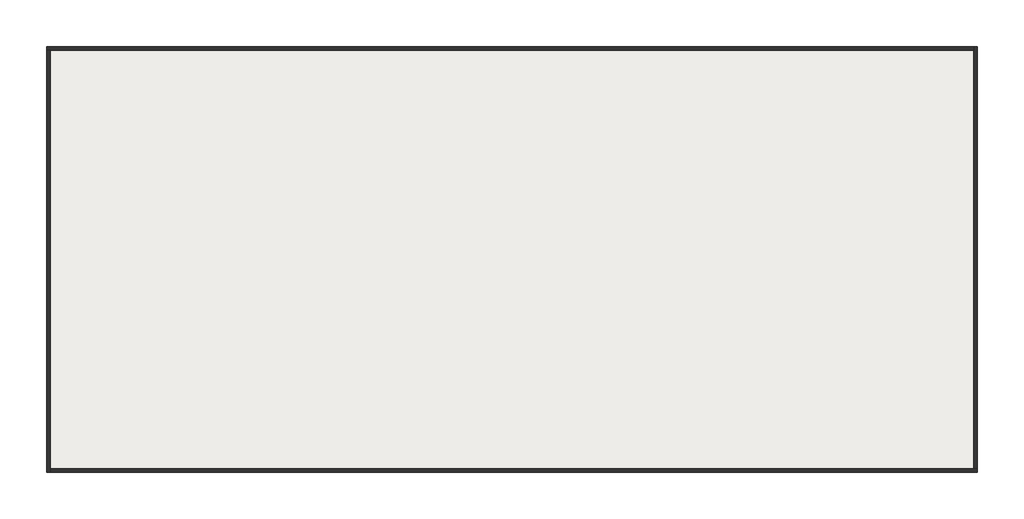
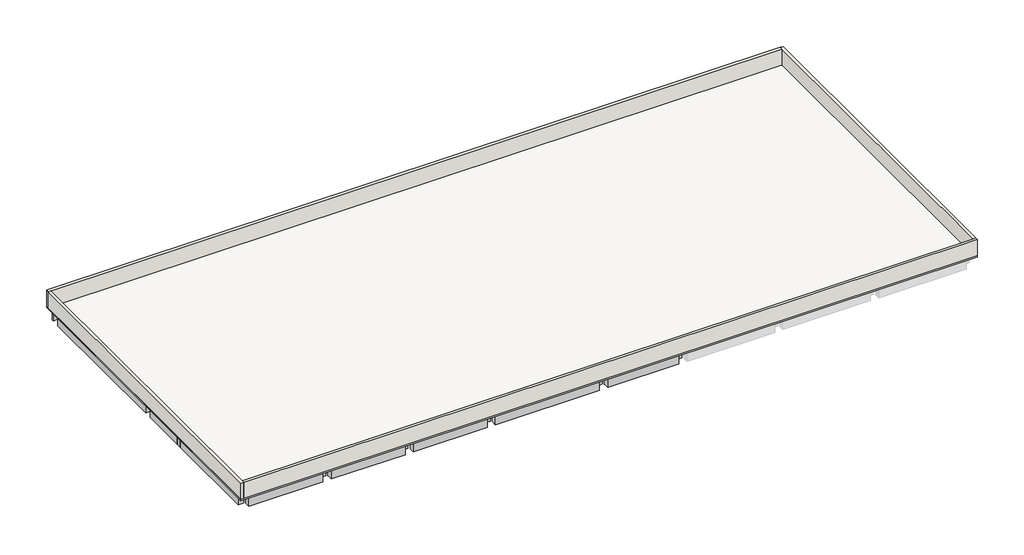
# One storey, part 1 of 2: 33 beams, 4 walls, 1 roof.
"""IFC4 building model written with IfcOpenShell, lengths in millimetres."""

from ifc_helpers import new_model, si_unit, frame, origin, place, context, project, spatial, polyline, outline, extrude, faceted_brep, element, save

model = new_model("IFC4")

# Units and contexts
model_context = context("Model", 3, world=origin())
ifc_project = project(units=[si_unit("LENGTHUNIT", "METRE", prefix="MILLI")], contexts=[model_context])

# Site, building, storey
site = spatial("IfcSite", under=ifc_project)
building = spatial("IfcBuilding", under=site)
storey = spatial("IfcBuildingStorey", under=building, Name="TOC", Elevation=7650.0)

# Beams
placement = place(None, origin())
element("IfcBeam", 1, ObjectType="RC Beam_Rectangular : H_SB_ACB_B400xH900", at=placement, inside=storey, context=model_context, shape_type="Brep", body=[
    faceted_brep([(224.7, 12116.5208589, 7500.0), (224.7, 12116.5208589, 6750.0), (5624.7, 12116.5208589, 6750.0), (5624.7, 12116.5208589, 7500.0), (5724.7, 12116.5208589, 7500.0), (6124.7, 12116.5208589, 7500.0), (6124.7, 12116.5208589, 7549.0), (5724.7, 12116.5208589, 7549.0), (124.7, 12116.5208589, 7549.0), (-275.3, 12116.5208589, 7549.0), (-275.3, 12116.5208589, 7500.0), (124.7, 12116.5208589, 7500.0), (224.7, 12199.5208589, 6750.0), (224.7, 12433.5208589, 6750.0), (224.7, 12516.5208589, 6750.0), (5624.7, 12516.5208589, 6750.0), (5624.7, 12433.5208589, 6750.0), (5624.7, 12199.5208589, 6750.0), (224.7, 12516.5208589, 7500.0), (124.7, 12516.5208589, 7500.0), (-275.3, 12516.5208589, 7500.0), (-275.3, 12516.5208589, 7549.0), (124.7, 12516.5208589, 7549.0), (5724.7, 12516.5208589, 7549.0), (6124.7, 12516.5208589, 7549.0), (6124.7, 12516.5208589, 7500.0), (5724.7, 12516.5208589, 7500.0), (5624.7, 12516.5208589, 7500.0)], [[[0, 1, 2, 3, 4, 5, 6, 7, 8, 9, 10, 11]], [[1, 12, 13, 14, 15, 16, 17, 2]], [[14, 18, 19, 20, 21, 22, 23, 24, 25, 26, 27, 15]], [[1, 0, 18, 14, 13, 12]], [[0, 11, 10, 20, 19, 18]], [[27, 3, 2, 17, 16, 15]], [[3, 27, 26, 25, 5, 4]], [[9, 8, 7, 6, 24, 23, 22, 21]], [[9, 21, 20, 10]], [[24, 6, 5, 25]]]),
])
element("IfcBeam", 2, ObjectType="RC Beam_Rectangular : H_SB_ACB_B400xH900", at=placement, inside=storey, context=model_context, shape_type="Brep", body=[
    faceted_brep([(6224.7, 12116.5208589, 7500.0), (6224.7, 12116.5208589, 6750.0), (11624.7, 12116.5208589, 6750.0), (11624.7, 12116.5208589, 7500.0), (11724.7, 12116.5208589, 7500.0), (12124.7, 12116.5208589, 7500.0), (12124.7, 12116.5208589, 7549.0), (11724.7, 12116.5208589, 7549.0), (6124.7, 12116.5208589, 7549.0), (6124.7, 12116.5208589, 7500.0), (6224.7, 12199.5208589, 6750.0), (6224.7, 12433.5208589, 6750.0), (6224.7, 12516.5208589, 6750.0), (11624.7, 12516.5208589, 6750.0), (11624.7, 12433.5208589, 6750.0), (11624.7, 12199.5208589, 6750.0), (6224.7, 12516.5208589, 7500.0), (6124.7, 12516.5208589, 7500.0), (6124.7, 12516.5208589, 7549.0), (11724.7, 12516.5208589, 7549.0), (12124.7, 12516.5208589, 7549.0), (12124.7, 12516.5208589, 7500.0), (11724.7, 12516.5208589, 7500.0), (11624.7, 12516.5208589, 7500.0)], [[[0, 1, 2, 3, 4, 5, 6, 7, 8, 9]], [[1, 10, 11, 12, 13, 14, 15, 2]], [[12, 16, 17, 18, 19, 20, 21, 22, 23, 13]], [[1, 0, 16, 12, 11, 10]], [[0, 9, 17, 16]], [[23, 3, 2, 15, 14, 13]], [[3, 23, 22, 21, 5, 4]], [[8, 7, 6, 20, 19, 18]], [[20, 6, 5, 21]], [[8, 18, 17, 9]]]),
])
element("IfcBeam", 3, ObjectType="RC Beam_Rectangular : H_SB_ACB_B400xH900", at=placement, inside=storey, context=model_context, shape_type="Brep", body=[
    faceted_brep([(12224.7, 12116.5208589, 7500.0), (12224.7, 12116.5208589, 6750.0), (17624.7, 12116.5208589, 6750.0), (17624.7, 12116.5208589, 7500.0), (17724.7, 12116.5208589, 7500.0), (18124.7, 12116.5208589, 7500.0), (18124.7, 12116.5208589, 7549.0), (17724.7, 12116.5208589, 7549.0), (12124.7, 12116.5208589, 7549.0), (12124.7, 12116.5208589, 7500.0), (12224.7, 12199.5208589, 6750.0), (12224.7, 12433.5208589, 6750.0), (12224.7, 12516.5208589, 6750.0), (17624.7, 12516.5208589, 6750.0), (17624.7, 12433.5208589, 6750.0), (17624.7, 12199.5208589, 6750.0), (12224.7, 12516.5208589, 7500.0), (12124.7, 12516.5208589, 7500.0), (12124.7, 12516.5208589, 7549.0), (17724.7, 12516.5208589, 7549.0), (18124.7, 12516.5208589, 7549.0), (18124.7, 12516.5208589, 7500.0), (17724.7, 12516.5208589, 7500.0), (17624.7, 12516.5208589, 7500.0)], [[[0, 1, 2, 3, 4, 5, 6, 7, 8, 9]], [[1, 10, 11, 12, 13, 14, 15, 2]], [[12, 16, 17, 18, 19, 20, 21, 22, 23, 13]], [[1, 0, 16, 12, 11, 10]], [[0, 9, 17, 16]], [[23, 3, 2, 15, 14, 13]], [[3, 23, 22, 21, 5, 4]], [[8, 7, 6, 20, 19, 18]], [[20, 6, 5, 21]], [[8, 18, 17, 9]]]),
])
element("IfcBeam", 4, ObjectType="RC Beam_Rectangular : H_SB_ACB_B400xH900", at=placement, inside=storey, context=model_context, shape_type="Brep", body=[
    faceted_brep([(26324.7, 12116.5208589, 7549.0), (25924.7, 12116.5208589, 7549.0), (18124.7, 12116.5208589, 7549.0), (18124.7, 12116.5208589, 7500.0), (18224.7, 12116.5208589, 7500.0), (18224.7, 12116.5208589, 6750.0), (25924.7, 12116.5208589, 6750.0), (26324.7, 12116.5208589, 6750.0), (26324.7, 12516.5208589, 6750.0), (18224.7, 12516.5208589, 6750.0), (25924.7, 12516.5208589, 6750.0), (18124.7, 12516.5208589, 7549.0), (25924.7, 12516.5208589, 7549.0), (26324.7, 12516.5208589, 7549.0), (18224.7, 12516.5208589, 7500.0), (18124.7, 12516.5208589, 7500.0)], [[[0, 1, 2, 3, 4, 5, 6, 7]], [[8, 7, 6, 5, 9, 10]], [[11, 12, 13, 8, 10, 9, 14, 15]], [[4, 14, 9, 5]], [[14, 4, 3, 15]], [[2, 1, 0, 13, 12, 11]], [[7, 8, 13, 0]], [[2, 11, 15, 3]]]),
])
element("IfcBeam", 5, ObjectType="RC Beam_Rectangular : H_SB_ACB_B400xH900", at=placement, inside=storey, context=model_context, shape_type="Brep", body=[
    faceted_brep([(32124.7, 12116.5208589, 6750.0), (32124.7, 12116.5208589, 7549.0), (31724.7, 12116.5208589, 7549.0), (26324.7, 12116.5208589, 7549.0), (26324.7, 12116.5208589, 6750.0), (31724.7, 12116.5208589, 6750.0), (32124.7, 12516.5208589, 6750.0), (26324.7, 12516.5208589, 6750.0), (31724.7, 12516.5208589, 6750.0), (32124.7, 12516.5208589, 7549.0), (26324.7, 12516.5208589, 7549.0), (31724.7, 12516.5208589, 7549.0)], [[[0, 1, 2, 3, 4, 5]], [[6, 0, 5, 4, 7, 8]], [[9, 6, 8, 7, 10, 11]], [[1, 9, 11, 10, 3, 2]], [[0, 6, 9, 1]], [[4, 3, 10, 7]]]),
])
element("IfcBeam", 6, ObjectType="RC Beam_Rectangular : H_SB_ACB_B400xH900", at=placement, inside=storey, context=model_context, shape_type="Brep", body=[
    faceted_brep([(224.7, 23816.5208589, 7500.0), (224.7, 23816.5208589, 6750.0), (5624.7, 23816.5208589, 6750.0), (5624.7, 23816.5208589, 7500.0), (5724.7, 23816.5208589, 7500.0), (5724.7, 23816.5208589, 7549.0), (124.7, 23816.5208589, 7549.0), (124.7, 23816.5208589, 7500.0), (224.7, 23886.5208589, 6750.0), (224.7, 24216.5208589, 6750.0), (5624.7, 24216.5208589, 6750.0), (5624.7, 23886.5208589, 6750.0), (224.7, 24216.5208589, 7500.0), (124.7, 24216.5208589, 7500.0), (124.7, 24216.5208589, 7549.0), (5724.7, 24216.5208589, 7549.0), (5724.7, 24216.5208589, 7500.0), (5624.7, 24216.5208589, 7500.0)], [[[0, 1, 2, 3, 4, 5, 6, 7]], [[1, 8, 9, 10, 11, 2]], [[9, 12, 13, 14, 15, 16, 17, 10]], [[1, 0, 12, 9, 8]], [[12, 0, 7, 13]], [[3, 2, 11, 10, 17]], [[3, 17, 16, 4]], [[14, 6, 5, 15]], [[7, 6, 14, 13]], [[5, 4, 16, 15]]]),
])
element("IfcBeam", 7, ObjectType="RC Beam_Rectangular : H_SB_ACB_B400xH900", at=placement, inside=storey, context=model_context, shape_type="Brep", body=[
    faceted_brep([(6224.7, 23816.5208589, 7500.0), (6224.7, 23816.5208589, 6750.0), (11624.7, 23816.5208589, 6750.0), (11624.7, 23816.5208589, 7500.0), (11724.7, 23816.5208589, 7500.0), (11724.7, 23816.5208589, 7549.0), (6124.7, 23816.5208589, 7549.0), (6124.7, 23816.5208589, 7500.0), (6224.7, 23886.5208589, 6750.0), (6224.7, 24216.5208589, 6750.0), (11624.7, 24216.5208589, 6750.0), (11624.7, 23886.5208589, 6750.0), (6224.7, 24216.5208589, 7500.0), (6124.7, 24216.5208589, 7500.0), (6124.7, 24216.5208589, 7549.0), (11724.7, 24216.5208589, 7549.0), (11724.7, 24216.5208589, 7500.0), (11624.7, 24216.5208589, 7500.0)], [[[0, 1, 2, 3, 4, 5, 6, 7]], [[1, 8, 9, 10, 11, 2]], [[9, 12, 13, 14, 15, 16, 17, 10]], [[1, 0, 12, 9, 8]], [[0, 7, 13, 12]], [[3, 2, 11, 10, 17]], [[3, 17, 16, 4]], [[14, 6, 5, 15]], [[6, 14, 13, 7]], [[5, 4, 16, 15]]]),
])
element("IfcBeam", 8, ObjectType="RC Beam_Rectangular : H_SB_ACB_B400xH900", at=placement, inside=storey, context=model_context, shape_type="Brep", body=[
    faceted_brep([(12224.7, 23816.5208589, 7500.0), (12224.7, 23816.5208589, 6750.0), (17624.7, 23816.5208589, 6750.0), (17624.7, 23816.5208589, 7500.0), (17724.7, 23816.5208589, 7500.0), (17724.7, 23816.5208589, 7549.0), (12124.7, 23816.5208589, 7549.0), (12124.7, 23816.5208589, 7500.0), (12224.7, 23886.5208589, 6750.0), (12224.7, 24216.5208589, 6750.0), (17624.7, 24216.5208589, 6750.0), (17624.7, 23886.5208589, 6750.0), (12224.7, 24216.5208589, 7500.0), (12124.7, 24216.5208589, 7500.0), (12124.7, 24216.5208589, 7549.0), (17724.7, 24216.5208589, 7549.0), (17724.7, 24216.5208589, 7500.0), (17624.7, 24216.5208589, 7500.0)], [[[0, 1, 2, 3, 4, 5, 6, 7]], [[1, 8, 9, 10, 11, 2]], [[9, 12, 13, 14, 15, 16, 17, 10]], [[1, 0, 12, 9, 8]], [[0, 7, 13, 12]], [[3, 2, 11, 10, 17]], [[3, 17, 16, 4]], [[14, 6, 5, 15]], [[6, 14, 13, 7]], [[5, 4, 16, 15]]]),
])
element("IfcBeam", 9, ObjectType="RC Beam_Rectangular : H_SB_ACB_B400xH900", at=placement, inside=storey, context=model_context, shape_type="Brep", body=[
    faceted_brep([(-275.3, 8216.5208589, 6750.0), (124.7, 8216.5208589, 6750.0), (5724.7, 8216.5208589, 6750.0), (6124.7, 8216.5208589, 6750.0), (6124.7, 8216.5208589, 7549.0), (5724.7, 8216.5208589, 7549.0), (124.7, 8216.5208589, 7549.0), (-275.3, 8216.5208589, 7549.0), (-275.3, 8616.5208589, 6750.0), (124.7, 8616.5208589, 6750.0), (5724.7, 8616.5208589, 6750.0), (6124.7, 8616.5208589, 6750.0), (-275.3, 8616.5208589, 7549.0), (124.7, 8616.5208589, 7549.0), (5724.7, 8616.5208589, 7549.0), (6124.7, 8616.5208589, 7549.0)], [[[0, 1, 2, 3, 4, 5, 6, 7]], [[0, 8, 9, 10, 11, 3, 2, 1]], [[11, 10, 9, 8, 12, 13, 14, 15]], [[7, 6, 5, 4, 15, 14, 13, 12]], [[8, 0, 7, 12]], [[3, 11, 15, 4]]]),
])
element("IfcBeam", 10, ObjectType="RC Beam_Rectangular : H_SB_ACB_B400xH900", at=placement, inside=storey, context=model_context, shape_type="Brep", body=[
    faceted_brep([(12124.7, 8216.5208589, 6750.0), (12124.7, 8216.5208589, 7549.0), (11724.7, 8216.5208589, 7549.0), (6124.7, 8216.5208589, 7549.0), (6124.7, 8216.5208589, 6750.0), (11724.7, 8216.5208589, 6750.0), (12124.7, 8616.5208589, 6750.0), (6124.7, 8616.5208589, 6750.0), (11724.7, 8616.5208589, 6750.0), (12124.7, 8616.5208589, 7549.0), (6124.7, 8616.5208589, 7549.0), (11724.7, 8616.5208589, 7549.0)], [[[0, 1, 2, 3, 4, 5]], [[6, 0, 5, 4, 7, 8]], [[9, 6, 8, 7, 10, 11]], [[1, 9, 11, 10, 3, 2]], [[0, 6, 9, 1]], [[4, 3, 10, 7]]]),
])
element("IfcBeam", 11, ObjectType="RC Beam_Rectangular : H_SB_ACB_B400xH900", at=placement, inside=storey, context=model_context, shape_type="Brep", body=[
    faceted_brep([(18124.7, 8216.5208589, 6750.0), (18124.7, 8216.5208589, 7549.0), (17724.7, 8216.5208589, 7549.0), (12124.7, 8216.5208589, 7549.0), (12124.7, 8216.5208589, 6750.0), (17724.7, 8216.5208589, 6750.0), (18124.7, 8616.5208589, 6750.0), (12124.7, 8616.5208589, 6750.0), (17724.7, 8616.5208589, 6750.0), (18124.7, 8616.5208589, 7549.0), (12124.7, 8616.5208589, 7549.0), (17724.7, 8616.5208589, 7549.0)], [[[0, 1, 2, 3, 4, 5]], [[6, 0, 5, 4, 7, 8]], [[9, 6, 8, 7, 10, 11]], [[1, 9, 11, 10, 3, 2]], [[0, 6, 9, 1]], [[4, 3, 10, 7]]]),
])
element("IfcBeam", 12, ObjectType="RC Beam_Rectangular : H_SB_ACB_B400xH900", at=placement, inside=storey, context=model_context, shape_type="Brep", body=[
    faceted_brep([(26324.7, 8216.5208589, 7549.0), (25924.7, 8216.5208589, 7549.0), (18124.7, 8216.5208589, 7549.0), (18124.7, 8216.5208589, 6750.0), (25824.7, 8216.5208589, 6750.0), (25824.7, 8216.5208589, 7500.0), (25924.7, 8216.5208589, 7500.0), (26324.7, 8216.5208589, 7500.0), (18124.7, 8616.5208589, 6750.0), (25824.7, 8616.5208589, 6750.0), (25824.7, 8533.5208589, 6750.0), (25824.7, 8299.5208589, 6750.0), (18124.7, 8616.5208589, 7549.0), (25924.7, 8616.5208589, 7549.0), (26324.7, 8616.5208589, 7549.0), (26324.7, 8616.5208589, 7500.0), (25924.7, 8616.5208589, 7500.0), (25824.7, 8616.5208589, 7500.0)], [[[0, 1, 2, 3, 4, 5, 6, 7]], [[3, 8, 9, 10, 11, 4]], [[12, 13, 14, 15, 16, 17, 9, 8]], [[17, 5, 4, 11, 10, 9]], [[5, 17, 16, 15, 7, 6]], [[2, 1, 0, 14, 13, 12]], [[14, 0, 7, 15]], [[3, 2, 12, 8]]]),
])
element("IfcBeam", 13, ObjectType="RC Beam_Rectangular : H_SB_ACB_B400xH900", at=placement, inside=storey, context=model_context, shape_type="Brep", body=[
    faceted_brep([(26424.7, 8216.5208589, 7500.0), (26424.7, 8216.5208589, 6750.0), (28824.7, 8216.5208589, 6750.0), (29058.7, 8216.5208589, 6750.0), (31624.7, 8216.5208589, 6750.0), (31624.7, 8216.5208589, 7500.0), (31724.7, 8216.5208589, 7500.0), (32124.7, 8216.5208589, 7500.0), (32124.7, 8216.5208589, 7549.0), (31724.7, 8216.5208589, 7549.0), (31624.7, 8216.5208589, 7549.0), (29058.7, 8216.5208589, 7549.0), (28824.7, 8216.5208589, 7549.0), (26424.7, 8216.5208589, 7549.0), (26324.7, 8216.5208589, 7549.0), (26324.7, 8216.5208589, 7500.0), (26424.7, 8299.5208589, 6750.0), (26424.7, 8533.5208589, 6750.0), (26424.7, 8616.5208589, 6750.0), (31624.7, 8616.5208589, 6750.0), (31624.7, 8533.5208589, 6750.0), (31624.7, 8299.5208589, 6750.0), (26424.7, 8616.5208589, 7500.0), (26324.7, 8616.5208589, 7500.0), (26324.7, 8616.5208589, 7549.0), (31724.7, 8616.5208589, 7549.0), (32124.7, 8616.5208589, 7549.0), (32124.7, 8616.5208589, 7500.0), (31724.7, 8616.5208589, 7500.0), (31624.7, 8616.5208589, 7500.0)], [[[0, 1, 2, 3, 4, 5, 6, 7, 8, 9, 10, 11, 12, 13, 14, 15]], [[1, 16, 17, 18, 19, 20, 21, 4, 3, 2]], [[18, 22, 23, 24, 25, 26, 27, 28, 29, 19]], [[1, 0, 22, 18, 17, 16]], [[0, 15, 23, 22]], [[29, 5, 4, 21, 20, 19]], [[5, 29, 28, 27, 7, 6]], [[14, 13, 12, 11, 10, 9, 8, 26, 25, 24]], [[26, 8, 7, 27]], [[14, 24, 23, 15]]]),
])
element("IfcBeam", 14, ObjectType="RC Beam_Rectangular : H_SB_ACB_B400xH900", at=placement, inside=storey, context=model_context, shape_type="Brep", body=[
    faceted_brep([(224.7, 416.5208589, 7500.0), (224.7, 416.5208589, 6750.0), (5624.7, 416.5208589, 6750.0), (5624.7, 416.5208589, 7500.0), (6124.7, 416.5208589, 7500.0), (6124.7, 416.5208589, 7549.0), (54.7, 416.5208589, 7549.0), (-275.3, 416.5208589, 7549.0), (-275.3, 416.5208589, 7500.0), (54.7, 416.5208589, 7500.0), (224.7, 746.5208589, 6750.0), (224.7, 816.5208589, 6750.0), (5624.7, 816.5208589, 6750.0), (5624.7, 746.5208589, 6750.0), (224.7, 816.5208589, 7500.0), (124.7, 816.5208589, 7500.0), (-275.3, 816.5208589, 7500.0), (-275.3, 816.5208589, 7549.0), (124.7, 816.5208589, 7549.0), (5724.7, 816.5208589, 7549.0), (6124.7, 816.5208589, 7549.0), (6124.7, 816.5208589, 7500.0), (5724.7, 816.5208589, 7500.0), (5624.7, 816.5208589, 7500.0)], [[[0, 1, 2, 3, 4, 5, 6, 7, 8, 9]], [[1, 10, 11, 12, 13, 2]], [[11, 14, 15, 16, 17, 18, 19, 20, 21, 22, 23, 12]], [[11, 10, 1, 0, 14]], [[16, 15, 14, 0, 9, 8]], [[23, 3, 2, 13, 12]], [[3, 23, 22, 21, 4]], [[7, 6, 5, 20, 19, 18, 17]], [[7, 17, 16, 8]], [[20, 5, 4, 21]]]),
])
element("IfcBeam", 15, ObjectType="RC Beam_Rectangular : H_SB_ACB_B400xH900", at=placement, inside=storey, context=model_context, shape_type="Brep", body=[
    faceted_brep([(6224.7, 416.5208589, 7500.0), (6224.7, 416.5208589, 6750.0), (11624.7, 416.5208589, 6750.0), (11624.7, 416.5208589, 7500.0), (12124.7, 416.5208589, 7500.0), (12124.7, 416.5208589, 7549.0), (6124.7, 416.5208589, 7549.0), (6124.7, 416.5208589, 7500.0), (6224.7, 746.5208589, 6750.0), (6224.7, 816.5208589, 6750.0), (11624.7, 816.5208589, 6750.0), (11624.7, 746.5208589, 6750.0), (6224.7, 816.5208589, 7500.0), (6124.7, 816.5208589, 7500.0), (6124.7, 816.5208589, 7549.0), (11724.7, 816.5208589, 7549.0), (12124.7, 816.5208589, 7549.0), (12124.7, 816.5208589, 7500.0), (11724.7, 816.5208589, 7500.0), (11624.7, 816.5208589, 7500.0)], [[[0, 1, 2, 3, 4, 5, 6, 7]], [[1, 8, 9, 10, 11, 2]], [[9, 12, 13, 14, 15, 16, 17, 18, 19, 10]], [[9, 8, 1, 0, 12]], [[13, 12, 0, 7]], [[19, 3, 2, 11, 10]], [[3, 19, 18, 17, 4]], [[6, 5, 16, 15, 14]], [[16, 5, 4, 17]], [[6, 14, 13, 7]]]),
])
element("IfcBeam", 16, ObjectType="RC Beam_Rectangular : H_SB_ACB_B400xH900", at=placement, inside=storey, context=model_context, shape_type="Brep", body=[
    faceted_brep([(12224.7, 416.5208589, 7500.0), (12224.7, 416.5208589, 6750.0), (17624.7, 416.5208589, 6750.0), (17624.7, 416.5208589, 7500.0), (18124.7, 416.5208589, 7500.0), (18124.7, 416.5208589, 7549.0), (12124.7, 416.5208589, 7549.0), (12124.7, 416.5208589, 7500.0), (12224.7, 746.5208589, 6750.0), (12224.7, 816.5208589, 6750.0), (17624.7, 816.5208589, 6750.0), (17624.7, 746.5208589, 6750.0), (12224.7, 816.5208589, 7500.0), (12124.7, 816.5208589, 7500.0), (12124.7, 816.5208589, 7549.0), (17724.7, 816.5208589, 7549.0), (18124.7, 816.5208589, 7549.0), (18124.7, 816.5208589, 7500.0), (17724.7, 816.5208589, 7500.0), (17624.7, 816.5208589, 7500.0)], [[[0, 1, 2, 3, 4, 5, 6, 7]], [[1, 8, 9, 10, 11, 2]], [[9, 12, 13, 14, 15, 16, 17, 18, 19, 10]], [[9, 8, 1, 0, 12]], [[13, 12, 0, 7]], [[19, 3, 2, 11, 10]], [[3, 19, 18, 17, 4]], [[6, 5, 16, 15, 14]], [[16, 5, 4, 17]], [[6, 14, 13, 7]]]),
])
element("IfcBeam", 17, ObjectType="RC Beam_Rectangular : H_SB_ACB_B400xH900", at=placement, inside=storey, context=model_context, shape_type="Brep", body=[
    faceted_brep([(18224.7, 416.5208589, 7500.0), (18224.7, 416.5208589, 6750.0), (25824.7, 416.5208589, 6750.0), (25824.7, 416.5208589, 7500.0), (26324.7, 416.5208589, 7500.0), (26324.7, 416.5208589, 7549.0), (18124.7, 416.5208589, 7549.0), (18124.7, 416.5208589, 7500.0), (18224.7, 746.5208589, 6750.0), (18224.7, 816.5208589, 6750.0), (25824.7, 816.5208589, 6750.0), (25824.7, 746.5208589, 6750.0), (18224.7, 816.5208589, 7500.0), (18124.7, 816.5208589, 7500.0), (18124.7, 816.5208589, 7549.0), (25924.7, 816.5208589, 7549.0), (26324.7, 816.5208589, 7549.0), (26324.7, 816.5208589, 7500.0), (25924.7, 816.5208589, 7500.0), (25824.7, 816.5208589, 7500.0)], [[[0, 1, 2, 3, 4, 5, 6, 7]], [[1, 8, 9, 10, 11, 2]], [[9, 12, 13, 14, 15, 16, 17, 18, 19, 10]], [[9, 8, 1, 0, 12]], [[13, 12, 0, 7]], [[19, 3, 2, 11, 10]], [[3, 19, 18, 17, 4]], [[6, 5, 16, 15, 14]], [[16, 5, 4, 17]], [[6, 14, 13, 7]]]),
])
element("IfcBeam", 18, ObjectType="RC Beam_Rectangular : H_SB_ACB_B400xH900", at=placement, inside=storey, context=model_context, shape_type="Brep", body=[
    faceted_brep([(26424.7, 416.5208589, 7500.0), (26424.7, 416.5208589, 6750.0), (31624.7, 416.5208589, 6750.0), (31624.7, 416.5208589, 7500.0), (32124.7, 416.5208589, 7500.0), (32124.7, 416.5208589, 7549.0), (26324.7, 416.5208589, 7549.0), (26324.7, 416.5208589, 7500.0), (26424.7, 746.5208589, 6750.0), (26424.7, 816.5208589, 6750.0), (28824.7, 816.5208589, 6750.0), (29058.7, 816.5208589, 6750.0), (31624.7, 816.5208589, 6750.0), (31624.7, 746.5208589, 6750.0), (26424.7, 816.5208589, 7500.0), (26324.7, 816.5208589, 7500.0), (26324.7, 816.5208589, 7549.0), (26424.7, 816.5208589, 7549.0), (28824.7, 816.5208589, 7549.0), (29058.7, 816.5208589, 7549.0), (31624.7, 816.5208589, 7549.0), (31724.7, 816.5208589, 7549.0), (32124.7, 816.5208589, 7549.0), (32124.7, 816.5208589, 7500.0), (31724.7, 816.5208589, 7500.0), (31624.7, 816.5208589, 7500.0)], [[[0, 1, 2, 3, 4, 5, 6, 7]], [[1, 8, 9, 10, 11, 12, 13, 2]], [[9, 14, 15, 16, 17, 18, 19, 20, 21, 22, 23, 24, 25, 12, 11, 10]], [[9, 8, 1, 0, 14]], [[15, 14, 0, 7]], [[25, 3, 2, 13, 12]], [[3, 25, 24, 23, 4]], [[6, 5, 22, 21, 20, 19, 18, 17, 16]], [[22, 5, 4, 23]], [[6, 16, 15, 7]]]),
])
element("IfcBeam", 19, ObjectType="RC Beam_Rectangular : H_SB_ACB_B400xH900", at=placement, inside=storey, context=model_context, shape_type="Brep", body=[
    faceted_brep([(124.7, 8216.5208589, 6750.0), (124.7, 8216.5208589, 7549.0), (124.7, 816.5208589, 7549.0), (124.7, 816.5208589, 7500.0), (124.7, 916.5208589, 7500.0), (124.7, 916.5208589, 6750.0), (-275.3, 8216.5208589, 6750.0), (54.7, 916.5208589, 6750.0), (-275.3, 916.5208589, 6750.0), (-275.3, 8216.5208589, 7549.0), (-275.3, 916.5208589, 7500.0), (-275.3, 816.5208589, 7500.0), (-275.3, 816.5208589, 7549.0)], [[[0, 1, 2, 3, 4, 5]], [[6, 0, 5, 7, 8]], [[9, 6, 8, 10, 11, 12]], [[1, 0, 6, 9]], [[2, 12, 11, 3]], [[4, 10, 8, 7, 5]], [[10, 4, 3, 11]], [[1, 9, 12, 2]]]),
])
element("IfcBeam", 20, ObjectType="RC Beam_Rectangular : H_SB_ACB_B400xH900", at=placement, inside=storey, context=model_context, shape_type="Brep", body=[
    faceted_brep([(124.7, 8616.5208589, 7549.0), (124.7, 8616.5208589, 6750.0), (124.7, 12016.5208589, 6750.0), (124.7, 12016.5208589, 7500.0), (124.7, 12116.5208589, 7500.0), (124.7, 12116.5208589, 7549.0), (-275.3, 8616.5208589, 6750.0), (-275.3, 12016.5208589, 6750.0), (54.7, 12016.5208589, 6750.0), (-275.3, 8616.5208589, 7549.0), (-275.3, 12116.5208589, 7549.0), (-275.3, 12116.5208589, 7500.0), (-275.3, 12016.5208589, 7500.0)], [[[0, 1, 2, 3, 4, 5]], [[1, 6, 7, 8, 2]], [[9, 10, 11, 12, 7, 6]], [[10, 5, 4, 11]], [[1, 0, 9, 6]], [[12, 3, 2, 8, 7]], [[3, 12, 11, 4]], [[5, 10, 9, 0]]]),
])
element("IfcBeam", 21, ObjectType="RC Beam_Rectangular : H_SB_ACB_B400xH900", at=placement, inside=storey, context=model_context, shape_type="Brep", body=[
    faceted_brep([(124.7, 24429.2208589, 6750.0), (-275.3, 24429.2208589, 6750.0), (-275.3, 24429.2208589, 7549.0), (124.7, 24429.2208589, 7549.0), (124.7, 12616.5208589, 7500.0), (124.7, 12616.5208589, 6750.0), (124.7, 23716.5208589, 6750.0), (124.7, 23716.5208589, 7500.0), (124.7, 23816.5208589, 7500.0), (124.7, 24216.5208589, 7500.0), (124.7, 24316.5208589, 7500.0), (124.7, 24316.5208589, 6750.0), (124.7, 24316.5208589, 7549.0), (124.7, 24216.5208589, 7549.0), (124.7, 23816.5208589, 7549.0), (124.7, 12516.5208589, 7549.0), (124.7, 12516.5208589, 7500.0), (-275.3, 24316.5208589, 6750.0), (-275.3, 12616.5208589, 6750.0), (-275.3, 12616.5208589, 7500.0), (-275.3, 12516.5208589, 7500.0), (-275.3, 12516.5208589, 7549.0), (-275.3, 23886.5208589, 7549.0), (-275.3, 24316.5208589, 7549.0), (-275.3, 24316.5208589, 7500.0), (-275.3, 23886.5208589, 7500.0), (-275.3, 23716.5208589, 7500.0), (-275.3, 23716.5208589, 6750.0), (54.7, 12616.5208589, 6750.0), (54.7, 23716.5208589, 6750.0)], [[[0, 1, 2, 3]], [[4, 5, 6, 7, 8, 9, 10, 11, 0, 3, 12, 13, 14, 15, 16]], [[1, 0, 11, 17]], [[18, 19, 20, 21, 22, 23, 2, 1, 17, 24, 25, 26, 27]], [[20, 16, 15, 21]], [[5, 4, 19, 18, 28]], [[4, 16, 20, 19]], [[26, 7, 6, 29, 27]], [[7, 26, 25, 24, 10, 9, 8]], [[3, 2, 23, 22, 21, 15, 14, 13, 12]], [[10, 24, 17, 11]], [[5, 28, 18, 27, 29, 6]]]),
])
element("IfcBeam", 22, ObjectType="RC Beam_Rectangular : H_SB_ACB_B400xH900", at=placement, inside=storey, context=model_context, shape_type="SweptSolid", body=[
    extrude(outline(polyline([(8216.5208589, 7549.0), (8216.5208589, 6750.0), (916.5208589, 6750.0), (916.5208589, 7500.0), (816.5208589, 7500.0), (816.5208589, 7549.0), (8216.5208589, 7549.0)])), frame((5724.7, 0.0, 0.0), z_axis=(1.0, 0.0, 0.0), x_axis=(0.0, 1.0, 0.0)), (0.0, 0.0, 1.0), 400.0),
])
element("IfcBeam", 23, ObjectType="RC Beam_Rectangular : H_SB_ACB_B400xH900", at=placement, inside=storey, context=model_context, shape_type="SweptSolid", body=[
    extrude(outline(polyline([(8616.5208589, 6750.0), (8616.5208589, 7549.0), (12116.5208589, 7549.0), (12116.5208589, 7500.0), (12016.5208589, 7500.0), (12016.5208589, 6750.0), (8616.5208589, 6750.0)])), frame((5724.7, 0.0, 0.0), z_axis=(1.0, 0.0, 0.0), x_axis=(0.0, 1.0, 0.0)), (0.0, 0.0, 1.0), 400.0),
])
element("IfcBeam", 24, ObjectType="RC Beam_Rectangular : H_SB_ACB_B400xH900", at=placement, inside=storey, context=model_context, shape_type="Brep", body=[
    faceted_brep([(6124.7, 24429.2208589, 6750.0), (5724.7, 24429.2208589, 6750.0), (5724.7, 24429.2208589, 7549.0), (6124.7, 24429.2208589, 7549.0), (6124.7, 12616.5208589, 7500.0), (6124.7, 12616.5208589, 6750.0), (6124.7, 23716.5208589, 6750.0), (6124.7, 23716.5208589, 7500.0), (6124.7, 23816.5208589, 7500.0), (6124.7, 24216.5208589, 7500.0), (6124.7, 24316.5208589, 7500.0), (6124.7, 24316.5208589, 6750.0), (6124.7, 24316.5208589, 7549.0), (6124.7, 24216.5208589, 7549.0), (6124.7, 23816.5208589, 7549.0), (6124.7, 12516.5208589, 7549.0), (6124.7, 12516.5208589, 7500.0), (5724.7, 24316.5208589, 6750.0), (5724.7, 24316.5208589, 7500.0), (5724.7, 24216.5208589, 7500.0), (5724.7, 23816.5208589, 7500.0), (5724.7, 23716.5208589, 7500.0), (5724.7, 23716.5208589, 6750.0), (5724.7, 12616.5208589, 6750.0), (5724.7, 12616.5208589, 7500.0), (5724.7, 12516.5208589, 7500.0), (5724.7, 12516.5208589, 7549.0), (5724.7, 23816.5208589, 7549.0), (5724.7, 24216.5208589, 7549.0), (5724.7, 24316.5208589, 7549.0)], [[[0, 1, 2, 3]], [[4, 5, 6, 7, 8, 9, 10, 11, 0, 3, 12, 13, 14, 15, 16]], [[1, 0, 11, 17]], [[2, 1, 17, 18, 19, 20, 21, 22, 23, 24, 25, 26, 27, 28, 29]], [[25, 16, 15, 26]], [[5, 4, 24, 23]], [[4, 16, 25, 24]], [[21, 7, 6, 22]], [[7, 21, 20, 19, 18, 10, 9, 8]], [[3, 2, 29, 28, 27, 26, 15, 14, 13, 12]], [[10, 18, 17, 11]], [[5, 23, 22, 6]]]),
])
element("IfcBeam", 25, ObjectType="RC Beam_Rectangular : H_SB_ACB_B400xH900", at=placement, inside=storey, context=model_context, shape_type="SweptSolid", body=[
    extrude(outline(polyline([(8216.5208589, 7549.0), (8216.5208589, 6750.0), (916.5208589, 6750.0), (916.5208589, 7500.0), (816.5208589, 7500.0), (816.5208589, 7549.0), (8216.5208589, 7549.0)])), frame((11724.7, 0.0, 0.0), z_axis=(1.0, 0.0, 0.0), x_axis=(0.0, 1.0, 0.0)), (0.0, 0.0, 1.0), 400.0),
])
element("IfcBeam", 26, ObjectType="RC Beam_Rectangular : H_SB_ACB_B400xH900", at=placement, inside=storey, context=model_context, shape_type="SweptSolid", body=[
    extrude(outline(polyline([(8616.5208589, 6750.0), (8616.5208589, 7549.0), (12116.5208589, 7549.0), (12116.5208589, 7500.0), (12016.5208589, 7500.0), (12016.5208589, 6750.0), (8616.5208589, 6750.0)])), frame((11724.7, 0.0, 0.0), z_axis=(1.0, 0.0, 0.0), x_axis=(0.0, 1.0, 0.0)), (0.0, 0.0, 1.0), 400.0),
])
element("IfcBeam", 27, ObjectType="RC Beam_Rectangular : H_SB_ACB_B400xH900", at=placement, inside=storey, context=model_context, shape_type="Brep", body=[
    faceted_brep([(12124.7, 24429.2208589, 6750.0), (11724.7, 24429.2208589, 6750.0), (11724.7, 24429.2208589, 7549.0), (12124.7, 24429.2208589, 7549.0), (12124.7, 12616.5208589, 7500.0), (12124.7, 12616.5208589, 6750.0), (12124.7, 23716.5208589, 6750.0), (12124.7, 23716.5208589, 7500.0), (12124.7, 23816.5208589, 7500.0), (12124.7, 24216.5208589, 7500.0), (12124.7, 24316.5208589, 7500.0), (12124.7, 24316.5208589, 6750.0), (12124.7, 24316.5208589, 7549.0), (12124.7, 24216.5208589, 7549.0), (12124.7, 23816.5208589, 7549.0), (12124.7, 12516.5208589, 7549.0), (12124.7, 12516.5208589, 7500.0), (11724.7, 24316.5208589, 6750.0), (11724.7, 24316.5208589, 7500.0), (11724.7, 24216.5208589, 7500.0), (11724.7, 23816.5208589, 7500.0), (11724.7, 23716.5208589, 7500.0), (11724.7, 23716.5208589, 6750.0), (11724.7, 12616.5208589, 6750.0), (11724.7, 12616.5208589, 7500.0), (11724.7, 12516.5208589, 7500.0), (11724.7, 12516.5208589, 7549.0), (11724.7, 23816.5208589, 7549.0), (11724.7, 24216.5208589, 7549.0), (11724.7, 24316.5208589, 7549.0)], [[[0, 1, 2, 3]], [[4, 5, 6, 7, 8, 9, 10, 11, 0, 3, 12, 13, 14, 15, 16]], [[1, 0, 11, 17]], [[2, 1, 17, 18, 19, 20, 21, 22, 23, 24, 25, 26, 27, 28, 29]], [[25, 16, 15, 26]], [[5, 4, 24, 23]], [[4, 16, 25, 24]], [[21, 7, 6, 22]], [[7, 21, 20, 19, 18, 10, 9, 8]], [[3, 2, 29, 28, 27, 26, 15, 14, 13, 12]], [[10, 18, 17, 11]], [[5, 23, 22, 6]]]),
])
element("IfcBeam", 28, ObjectType="RC Beam_Rectangular : H_SB_ACB_B400xH900", at=placement, inside=storey, context=model_context, shape_type="Brep", body=[
    faceted_brep([(18124.7, 8216.5208589, 6750.0), (18124.7, 8216.5208589, 7549.0), (18124.7, 816.5208589, 7549.0), (18124.7, 816.5208589, 7500.0), (18124.7, 916.5208589, 7500.0), (18124.7, 916.5208589, 6750.0), (17724.7, 8216.5208589, 6750.0), (18041.7, 916.5208589, 6750.0), (17807.7, 916.5208589, 6750.0), (17724.7, 916.5208589, 6750.0), (17724.7, 8216.5208589, 7549.0), (17724.7, 916.5208589, 7500.0), (17724.7, 816.5208589, 7500.0), (17724.7, 816.5208589, 7549.0)], [[[0, 1, 2, 3, 4, 5]], [[6, 0, 5, 7, 8, 9]], [[10, 6, 9, 11, 12, 13]], [[0, 6, 10, 1]], [[2, 13, 12, 3]], [[4, 11, 9, 8, 7, 5]], [[11, 4, 3, 12]], [[1, 10, 13, 2]]]),
])
element("IfcBeam", 29, ObjectType="RC Beam_Rectangular : H_SB_ACB_B400xH900", at=placement, inside=storey, context=model_context, shape_type="Brep", body=[
    faceted_brep([(18124.7, 12116.5208589, 7549.0), (18124.7, 8616.5208589, 7549.0), (18124.7, 8616.5208589, 6750.0), (18124.7, 12016.5208589, 6750.0), (18124.7, 12016.5208589, 7500.0), (18124.7, 12116.5208589, 7500.0), (17724.7, 8616.5208589, 6750.0), (17724.7, 12016.5208589, 6750.0), (17807.7, 12016.5208589, 6750.0), (18041.7, 12016.5208589, 6750.0), (17724.7, 8616.5208589, 7549.0), (17724.7, 12116.5208589, 7549.0), (17724.7, 12116.5208589, 7500.0), (17724.7, 12016.5208589, 7500.0)], [[[0, 1, 2, 3, 4, 5]], [[2, 6, 7, 8, 9, 3]], [[6, 10, 11, 12, 13, 7]], [[11, 0, 5, 12]], [[6, 2, 1, 10]], [[13, 4, 3, 9, 8, 7]], [[4, 13, 12, 5]], [[0, 11, 10, 1]]]),
])
element("IfcBeam", 30, ObjectType="RC Beam_Rectangular : H_SB_ACB_B400xH900", at=placement, inside=storey, context=model_context, shape_type="Brep", body=[
    faceted_brep([(26324.7, 8116.5208589, 6750.0), (26324.7, 8116.5208589, 7500.0), (26324.7, 8216.5208589, 7500.0), (26324.7, 8216.5208589, 7549.0), (26324.7, 816.5208589, 7549.0), (26324.7, 816.5208589, 7500.0), (26324.7, 916.5208589, 7500.0), (26324.7, 916.5208589, 6750.0), (25924.7, 8116.5208589, 6750.0), (26190.7, 8116.5208589, 6750.0), (26190.7, 916.5208589, 6750.0), (25924.7, 916.5208589, 6750.0), (25924.7, 8116.5208589, 7500.0), (25924.7, 916.5208589, 7500.0), (25924.7, 816.5208589, 7500.0), (25924.7, 816.5208589, 7549.0), (25924.7, 8216.5208589, 7549.0), (25924.7, 8216.5208589, 7500.0)], [[[0, 1, 2, 3, 4, 5, 6, 7]], [[8, 9, 0, 7, 10, 11]], [[12, 8, 11, 13, 14, 15, 16, 17]], [[2, 17, 16, 3]], [[4, 15, 14, 5]], [[1, 0, 9, 8, 12]], [[2, 1, 12, 17]], [[6, 13, 11, 10, 7]], [[13, 6, 5, 14]], [[3, 16, 15, 4]]]),
])
element("IfcBeam", 31, ObjectType="RC Beam_Rectangular : H_SB_ACB_B400xH900", at=placement, inside=storey, context=model_context, shape_type="SweptSolid", body=[
    extrude(outline(polyline([(12116.5208589, 7549.0), (12116.5208589, 6750.0), (8716.5208589, 6750.0), (8716.5208589, 7500.0), (8616.5208589, 7500.0), (8616.5208589, 7549.0), (12116.5208589, 7549.0)])), frame((25924.7, 0.0, 0.0), z_axis=(1.0, 0.0, 0.0), x_axis=(0.0, 1.0, 0.0)), (0.0, 0.0, 1.0), 400.0),
])
element("IfcBeam", 32, ObjectType="RC Beam_Rectangular : H_SB_ACB_B400xH900", at=placement, inside=storey, context=model_context, shape_type="Brep", body=[
    faceted_brep([(32124.7, 8116.5208589, 6750.0), (32124.7, 8116.5208589, 7500.0), (32124.7, 8216.5208589, 7500.0), (32124.7, 8216.5208589, 7549.0), (32124.7, 816.5208589, 7549.0), (32124.7, 816.5208589, 7500.0), (32124.7, 916.5208589, 7500.0), (32124.7, 916.5208589, 6750.0), (31724.7, 8116.5208589, 6750.0), (31858.7, 8116.5208589, 6750.0), (31858.7, 916.5208589, 6750.0), (31724.7, 916.5208589, 6750.0), (31724.7, 8116.5208589, 7500.0), (31724.7, 916.5208589, 7500.0), (31724.7, 816.5208589, 7500.0), (31724.7, 816.5208589, 7549.0), (31724.7, 8216.5208589, 7549.0), (31724.7, 8216.5208589, 7500.0)], [[[0, 1, 2, 3, 4, 5, 6, 7]], [[8, 9, 0, 7, 10, 11]], [[12, 8, 11, 13, 14, 15, 16, 17]], [[2, 17, 16, 3]], [[4, 15, 14, 5]], [[1, 0, 9, 8, 12]], [[2, 1, 12, 17]], [[6, 13, 11, 10, 7]], [[13, 6, 5, 14]], [[3, 16, 15, 4]]]),
])
element("IfcBeam", 33, ObjectType="RC Beam_Rectangular : H_SB_ACB_B400xH900", at=placement, inside=storey, context=model_context, shape_type="SweptSolid", body=[
    extrude(outline(polyline([(12116.5208589, 7549.0), (12116.5208589, 6750.0), (8716.5208589, 6750.0), (8716.5208589, 7500.0), (8616.5208589, 7500.0), (8616.5208589, 7549.0), (12116.5208589, 7549.0)])), frame((31724.7, 0.0, 0.0), z_axis=(1.0, 0.0, 0.0), x_axis=(0.0, 1.0, 0.0)), (0.0, 0.0, 1.0), 400.0),
])

# Roof
element("IfcRoof", 34, ObjectType="H_RF_AMF_RC Roof Finish_WP_Insulation_Protection", at=placement, inside=storey, context=model_context, shape_type="SweptSolid", body=[
    extrude(outline(polyline([(53324.7, 24816.5208589), (53324.7, 216.5208589), (-475.3, 216.5208589), (-475.3, 24816.5208589), (53324.7, 24816.5208589)])), frame((0.0, 0.0, 7549.0), z_axis=(0.0, 0.0, 1.0), x_axis=(1.0, 0.0, 0.0)), (0.0, 0.0, 1.0), 101.0),
])

# Walls
element("IfcWall", 35, ObjectType="H_WA_AMW_RC Wall_T200 (No Finish)", at=placement, inside=storey, context=model_context, shape_type="Brep", body=[
    faceted_brep([(-475.3, 24616.5208589, 7650.0), (-275.3, 24616.5208589, 7650.0), (53124.7, 24616.5208589, 7650.0), (53124.7, 24616.5208589, 8900.0), (-275.3, 24616.5208589, 8900.0), (-475.3, 24616.5208589, 8900.0), (-475.3, 24816.5208589, 7650.0), (-475.3, 24816.5208589, 8900.0), (53124.7, 24816.5208589, 8900.0), (53124.7, 24816.5208589, 7650.0)], [[[0, 1, 2, 3, 4, 5]], [[6, 7, 8, 9]], [[2, 1, 0, 6, 9]], [[5, 4, 3, 8, 7]], [[0, 5, 7, 6]], [[3, 2, 9, 8]]]),
])
element("IfcWall", 36, ObjectType="H_WA_AMW_RC Wall_T200 (No Finish)", at=placement, inside=storey, context=model_context, shape_type="Brep", body=[
    faceted_brep([(-275.3, 216.5208589, 7650.0), (-275.3, 416.5208589, 7650.0), (-275.3, 24616.5208589, 7650.0), (-275.3, 24616.5208589, 8900.0), (-275.3, 416.5208589, 8900.0), (-275.3, 216.5208589, 8900.0), (-475.3, 216.5208589, 7650.0), (-475.3, 216.5208589, 8900.0), (-475.3, 24616.5208589, 8900.0), (-475.3, 24616.5208589, 7650.0)], [[[0, 1, 2, 3, 4, 5]], [[6, 7, 8, 9]], [[2, 1, 0, 6, 9]], [[5, 4, 3, 8, 7]], [[0, 5, 7, 6]], [[3, 2, 9, 8]]]),
])
element("IfcWall", 37, ObjectType="H_WA_AMW_RC Wall_T200 (No Finish)", at=placement, inside=storey, context=model_context, shape_type="Brep", body=[
    faceted_brep([(53324.7, 416.5208589, 7650.0), (53124.7, 416.5208589, 7650.0), (-275.3, 416.5208589, 7650.0), (-275.3, 416.5208589, 8900.0), (53124.7, 416.5208589, 8900.0), (53324.7, 416.5208589, 8900.0), (53324.7, 216.5208589, 7650.0), (53324.7, 216.5208589, 8900.0), (-275.3, 216.5208589, 8900.0), (-275.3, 216.5208589, 7650.0)], [[[0, 1, 2, 3, 4, 5]], [[6, 7, 8, 9]], [[2, 1, 0, 6, 9]], [[5, 4, 3, 8, 7]], [[0, 5, 7, 6]], [[3, 2, 9, 8]]]),
])
element("IfcWall", 38, ObjectType="H_WA_AMW_RC Wall_T200 (No Finish)", at=placement, inside=storey, context=model_context, shape_type="Brep", body=[
    faceted_brep([(53124.7, 24816.5208589, 7650.0), (53124.7, 24616.5208589, 7650.0), (53124.7, 416.5208589, 7650.0), (53124.7, 416.5208589, 8900.0), (53124.7, 24616.5208589, 8900.0), (53124.7, 24816.5208589, 8900.0), (53324.7, 24816.5208589, 7650.0), (53324.7, 24816.5208589, 8900.0), (53324.7, 416.5208589, 8900.0), (53324.7, 416.5208589, 7650.0)], [[[0, 1, 2, 3, 4, 5]], [[6, 7, 8, 9]], [[2, 1, 0, 6, 9]], [[5, 4, 3, 8, 7]], [[0, 5, 7, 6]], [[3, 2, 9, 8]]]),
])

save(model, "model.ifc")

# Revit data of these elements
# Type "RC Beam_Rectangular : H_SB_ACB_B400xH900"
#   중앙부 하부근 = ""
#   중앙부 상부근 = ""
#   중앙부 보조근 = ""
#   중앙부 늑근 = ""
#   외단부 하부근 = ""
#   외단부 상부근 = ""
#   외단부 보조근 = ""
#   외단부 늑근 = ""
#   부호 = "TG3"
#   내단부 하부근 = ""
#   내단부 상부근 = ""
#   내단부 보조근 = ""
#   내단부 늑근 = ""
#   ALL 하부근 = "3-D20"
#   ALL 상부근 = "3-D20"
#   ALL 보조근 = ""
#   ALL 늑근 = "2-D10 @120"
#   Width = 400.000 mm
#   Height = 900.000 mm
#   Length [instance default] = 1524.000 mm
#   b = 400.000 mm
#   h = 900.000 mm
#   hec_material3 [instance default] = none
#   hec_material2 [instance default] = none
#   hec_material1 [instance default] = none
#   Structural Material [instance default] = none
#   Assembly Code = ""
# Type "H_RF_AMF_RC Roof Finish_WP_Insulation_Protection"
#   Layers, outside or top first: 50.000 mm no material (function 4); 0.000 mm no material (function 100); 50.000 mm no material (function 3); 1.000 mm no material (function 2)
# Type "H_WA_AMW_RC Wall_T200 (No Finish)"
#   Type Comments = ""
#   Layers, outside or top first: 0.000 mm no material (function 100); 0.000 mm no material (function 100); 200.000 mm no material (function 1); 0.000 mm no material (function 100); 0.000 mm no material (function 100); 0.000 mm no material (function 100)
# Elements 1, 2, 3, 4, 5, 6, 7, 8, 9, 10, 11, 12, 13, 14, 15, 16, 17, 18, 19, 20, 21, 22, 23, 24, 25, 26, 27, 28, 29, 30, 31, 32, 33 (IfcBeam, "RC Beam_Rectangular : H_SB_ACB_B400xH900")
#   hec_material3 = none
#   hec_material2 = none
#   hec_material1 = none
#   Structural Material = none
#   Phase Created = New Construction
# Element 34 (IfcRoof, "H_RF_AMF_RC Roof Finish_WP_Insulation_Protection")
#   Mark = "RF1"
#   Roof Style Name = "Lightweight Concrete(Slope)+Insulation+Waterproofing+Gravel"
#   Roof Ref. = ""
#   Roof Base Material = "Concrete Slab"
#   Roof Finish_1 = "Light-Weight Concrete Screed (Slope 1%)"
#   Roof Finish_2 = ""
#   Roof Finish_3 = "Rigid Extruded Polystyrene Foam Insulation(XPS)"
#   Roof Finish_4 = "Waterproofing Membrane-EPDM(or Equivalent)"
#   Roof Finish_5 = "Gravel for Roof"
#   built-in parameter 1001705 = 25.0984 (stored number, unit not read)
#   built-in parameter 1001701 = -0.331365 (stored number, unit not read)
#   built-in parameter 1001710 = 33615
#   Roof Style = RF13
#   Phase Created = New Construction
#   Materials on its faces: "Default Roof"
# Element 35 (IfcWall, "H_WA_AMW_RC Wall_T200 (No Finish)")
#   Mark = "PW1"
#   Wall Loca = "ROOF"
#   Wall Style Name = "Concrete Wall+Acrylic Emulsion Paint on Cement Plaster"
#   Wall Ref. = ""
#   Wall Base Material-1 = ""
#   Wall Base Material-2 = ""
#   Wall Base Material-3 = "Concrete Wall"
#   Wall Finish-Ex = "Acrylic Emulsion Paint on Fair Faced Concrete"
#   Top Offset = 0.000 mm
#   Base Offset = 0.000 mm
#   wall height = 1250.000 mm
#   Wall Style No = EW51
#   Phase Created = New Construction
#   Base Constraint = TOC
#   Top Constraint = TOP
#   Materials on its faces: "Default Wall"
# Element 36 (IfcWall, "H_WA_AMW_RC Wall_T200 (No Finish)")
#   Mark = "PW2"
#   Wall Loca = "ROOF"
#   Wall Style Name = "Concrete Wall+Acrylic Emulsion Paint on Cement Plaster"
#   Wall Ref. = ""
#   Wall Base Material-1 = ""
#   Wall Base Material-2 = ""
#   Wall Base Material-3 = "Concrete Wall"
#   Wall Finish-Ex = "Acrylic Emulsion Paint on Fair Faced Concrete"
#   Top Offset = 0.000 mm
#   Base Offset = 0.000 mm
#   wall height = 1250.000 mm
#   Wall Style No = EW51
#   Phase Created = New Construction
#   Base Constraint = TOC
#   Top Constraint = TOP
#   Materials on its faces: "Default Wall"
# Element 37 (IfcWall, "H_WA_AMW_RC Wall_T200 (No Finish)")
#   Mark = "PW3"
#   Wall Loca = "ROOF"
#   Wall Style Name = "Concrete Wall+Acrylic Emulsion Paint on Cement Plaster"
#   Wall Ref. = ""
#   Wall Base Material-1 = ""
#   Wall Base Material-2 = ""
#   Wall Base Material-3 = "Concrete Wall"
#   Wall Finish-Ex = "Acrylic Emulsion Paint on Fair Faced Concrete"
#   Top Offset = 0.000 mm
#   Base Offset = 0.000 mm
#   wall height = 1250.000 mm
#   Wall Style No = EW51
#   Phase Created = New Construction
#   Base Constraint = TOC
#   Top Constraint = TOP
#   Materials on its faces: "Default Wall"
# Element 38 (IfcWall, "H_WA_AMW_RC Wall_T200 (No Finish)")
#   Mark = "PW4"
#   Wall Loca = "ROOF"
#   Wall Style Name = "Concrete Wall+Acrylic Emulsion Paint on Cement Plaster"
#   Wall Ref. = ""
#   Wall Base Material-1 = ""
#   Wall Base Material-2 = ""
#   Wall Base Material-3 = "Concrete Wall"
#   Wall Finish-Ex = "Acrylic Emulsion Paint on Fair Faced Concrete"
#   Top Offset = 0.000 mm
#   Base Offset = 0.000 mm
#   wall height = 1250.000 mm
#   Wall Style No = EW51
#   Phase Created = New Construction
#   Base Constraint = TOC
#   Top Constraint = TOP
#   Materials on its faces: "Default Wall"
# Materials
#   "Default Roof": class "Miscellaneous", colour RGB 80 80 80, transparency 0
#   "Default Wall": class "Miscellaneous", colour RGB 80 80 80, transparency 0
